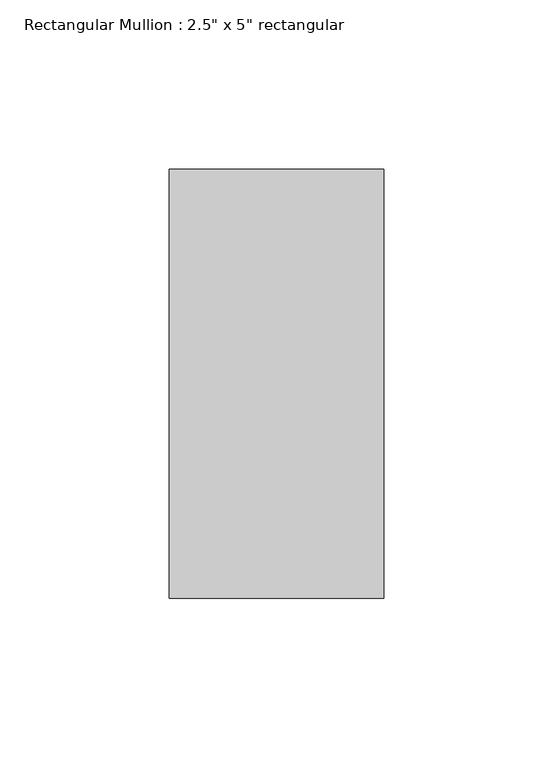
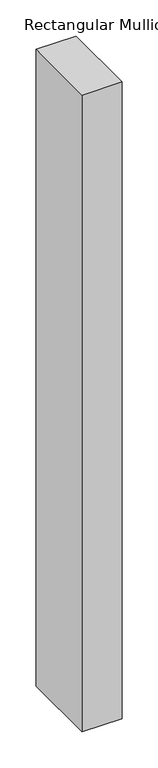
"""IFC4 building model written with IfcOpenShell, lengths in millimetres: member geometry."""

from ifc_helpers import new_model, si_unit, frame, origin, place, context, project, spatial, polyline, outline, extrude, source, transform, mapped, element, save


def member_9b1c5889(model_context):
    return source(origin(), model_context, "Body", "SweptSolid", [
        extrude(outline(polyline([(0.0, 63.5), (0.0, -63.5), (-63.5, -63.5), (-63.5, 63.5), (0.0, 63.5)])), frame((0.0, 0.0, -1073.1500001), z_axis=(0.0, 0.0, 1.0), x_axis=(1.0, 0.0, 0.0)), (0.0, 0.0, 1.0), 1073.1500001),
    ])


if __name__ == "__main__":
    model = new_model("IFC4")
    model_context = context("Model", 3, world=origin())
    ifc_project = project(units=[si_unit("LENGTHUNIT", "METRE", prefix="MILLI")], contexts=[model_context])
    site = spatial("IfcSite", under=ifc_project)
    building = spatial("IfcBuilding", under=site)
    placement = place(None, origin())
    member_shape = member_9b1c5889(model_context)
    element("IfcMember", 1, ObjectType="Rectangular Mullion : 2.5\" x 5\" rectangular", at=placement, inside=building, context=model_context, shape_type="MappedRepresentation", body=[
        mapped(member_shape, transform((0.0, 0.0, 0.0), x_axis=(1.0, 0.0, 0.0), y_axis=(0.0, 1.0, 0.0), z_axis=(0.0, 0.0, 1.0))),
    ])
    save(model, "model.ifc")

# Revit data of these elements
# Type "Rectangular Mullion : 2.5\" x 5\" rectangular"
#   built-in parameter 1007304 = 0.416667 (stored number, unit not read)
#   built-in parameter 1007301 = 0.104167 (stored number, unit not read)
#   built-in parameter 1007300 = 0.104167 (stored number, unit not read)
# Element 1 (IfcMember, "Rectangular Mullion : 2.5\" x 5\" rectangular")
#   Materials on its faces: "Aluminum"
# Materials
#   "Aluminum": class "Metal", colour RGB 247 247 247, transparency 0, Description = "Aluminum 6061", Cost = 0
